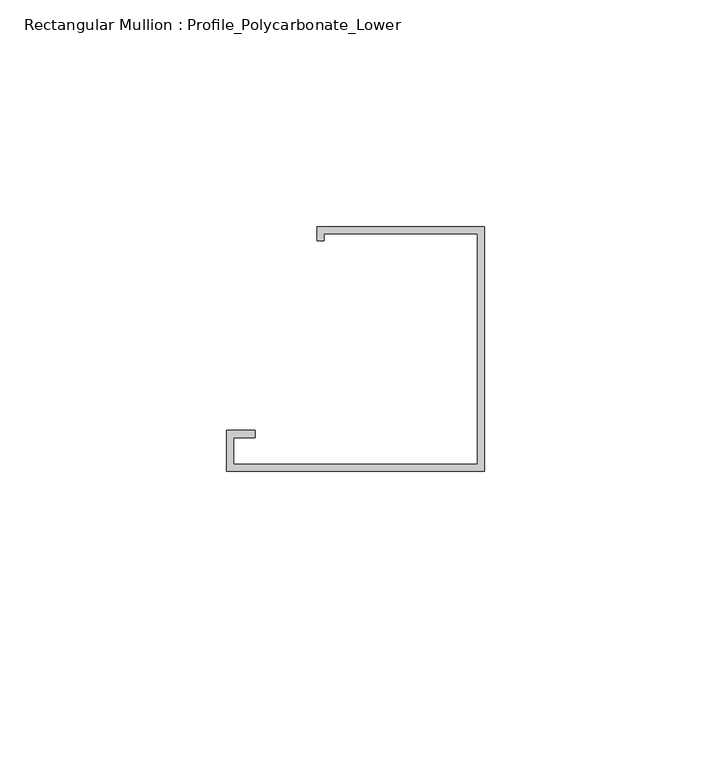
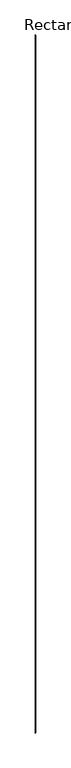
"""IFC4 building model written with IfcOpenShell, lengths in millimetres: member geometry, Rectangular Mullion : Profile_Polycarbonate_Lower."""

from ifc_helpers import new_model, si_unit, frame, origin, place, context, project, spatial, polyline, outline, extrude, source, transform, mapped, element, save


def rectangular_mullion_profile_polycarbonate_lower_d7ba2170(model_context):
    return source(origin(), model_context, "Body", "SweptSolid", [
        extrude(outline(polyline([(0.0, -28.984575), (-56.9976, -28.984575), (-56.9976, -19.992975), (-50.6476, -19.992975), (-50.6476, -21.580475), (-55.4101, -21.580475), (-55.4101, -27.397075), (-1.5875, -27.397075), (-1.5875, 23.428325), (-35.3949, 23.428325), (-35.3949, 21.840825), (-36.9824, 21.840825), (-36.9824, 25.015825), (0.0, 25.015825), (0.0, -28.984575)])), frame((0.0, 0.0, -88808.486975), z_axis=(0.0, 0.0, 1.0), x_axis=(1.0, 0.0, 0.0)), (0.0, 0.0, 1.0), 88808.486975),
    ])


if __name__ == "__main__":
    model = new_model("IFC4")
    model_context = context("Model", 3, world=origin())
    ifc_project = project(units=[si_unit("LENGTHUNIT", "METRE", prefix="MILLI")], contexts=[model_context])
    site = spatial("IfcSite", under=ifc_project)
    building = spatial("IfcBuilding", under=site)
    placement = place(None, origin())
    rectangular_mullion_profile_polycarbonate_lower_shape = rectangular_mullion_profile_polycarbonate_lower_d7ba2170(model_context)
    element("IfcMember", 1, ObjectType="Rectangular Mullion : Profile_Polycarbonate_Lower", at=placement, inside=building, context=model_context, shape_type="MappedRepresentation", body=[
        mapped(rectangular_mullion_profile_polycarbonate_lower_shape, transform((0.0, 0.0, 0.0), x_axis=(1.0, 0.0, 0.0), y_axis=(0.0, 1.0, 0.0), z_axis=(0.0, 0.0, 1.0))),
    ])
    save(model, "model.ifc")

# Revit data of these elements
# Type "Rectangular Mullion : Profile_Polycarbonate_Lower"
#   built-in parameter 1007322 = 0.177167 (stored number, unit not read)
#   built-in parameter 1007321 = 0 (stored number, unit not read)
#   built-in parameter 1007320 = 0.00520833 (stored number, unit not read)
